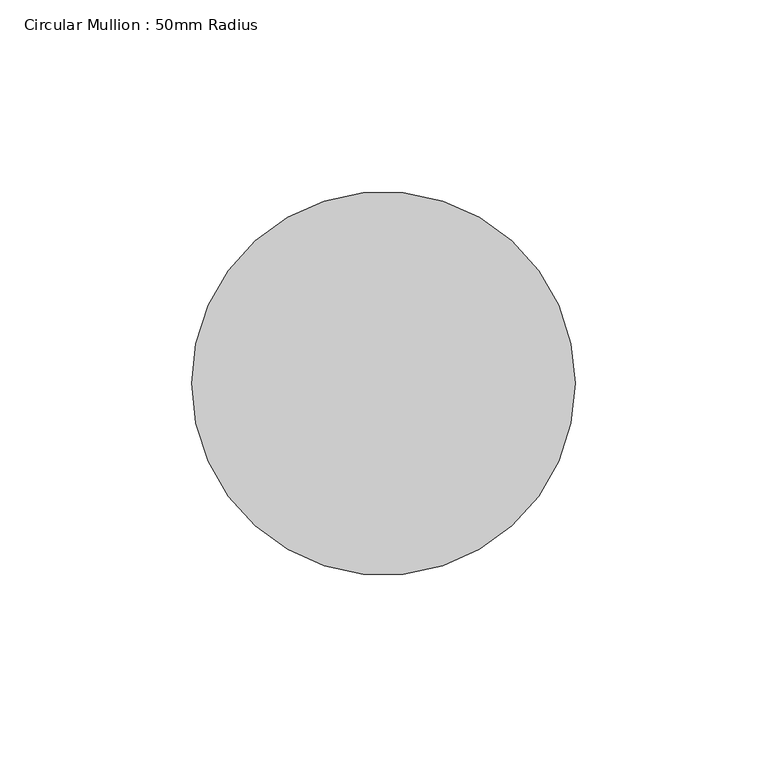
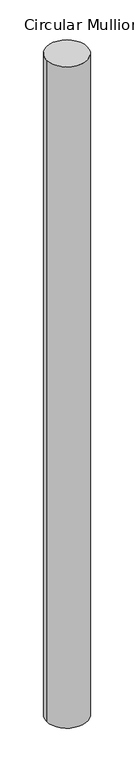
"""IFC4 building model written with IfcOpenShell, lengths in millimetres: member geometry, Circular Mullion : 50mm Radius."""

from ifc_helpers import new_model, si_unit, point, frame, origin, origin_2d, place, context, project, spatial, circle_curve, trimmed, segment, composite_curve, outline, extrude, source, transform, mapped, element, save


def circular_mullion_50mm_radius_2920e9e4(model_context):
    return source(origin(), model_context, "Body", "SweptSolid", [
        extrude(outline(composite_curve([segment(trimmed(circle_curve(origin_2d(), 50.0), [point((50.0, 0.0))], [point((-50.0, 0.0))], False, "CARTESIAN"), True, "CONTINUOUS"), segment(trimmed(circle_curve(origin_2d(), 50.0), [point((-50.0, 0.0))], [point((50.0, 0.0))], False, "CARTESIAN"), True, "CONTINUOUS")], self_intersect=False)), frame((0.0, 0.0, -1713.370382), z_axis=(0.0, 0.0, 1.0), x_axis=(1.0, 0.0, 0.0)), (0.0, 0.0, 1.0), 1713.370382),
    ])


if __name__ == "__main__":
    model = new_model("IFC4")
    model_context = context("Model", 3, world=origin())
    ifc_project = project(units=[si_unit("LENGTHUNIT", "METRE", prefix="MILLI")], contexts=[model_context])
    site = spatial("IfcSite", under=ifc_project)
    building = spatial("IfcBuilding", under=site)
    placement = place(None, origin())
    circular_mullion_50mm_radius_shape = circular_mullion_50mm_radius_2920e9e4(model_context)
    element("IfcMember", 1, ObjectType="Circular Mullion : 50mm Radius", at=placement, inside=building, context=model_context, shape_type="MappedRepresentation", body=[
        mapped(circular_mullion_50mm_radius_shape, transform((0.0, 0.0, 0.0), x_axis=(1.0, 0.0, 0.0), y_axis=(0.0, 1.0, 0.0), z_axis=(0.0, 0.0, 1.0))),
    ])
    save(model, "model.ifc")

# Revit data of these elements
# Type "Circular Mullion : 50mm Radius"
#   built-in parameter 1007350 = 0.164042 (stored number, unit not read)
# Element 1 (IfcMember, "Circular Mullion : 50mm Radius")
#   Materials on its faces: "Aluminium"
# Materials
#   "Aluminium": class "Metal", colour RGB 247 247 247, transparency 0, Description = "Aluminium 6061", Cost = 0
